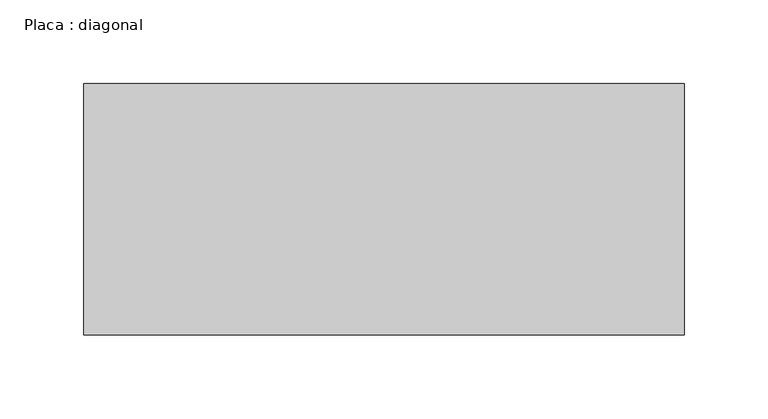
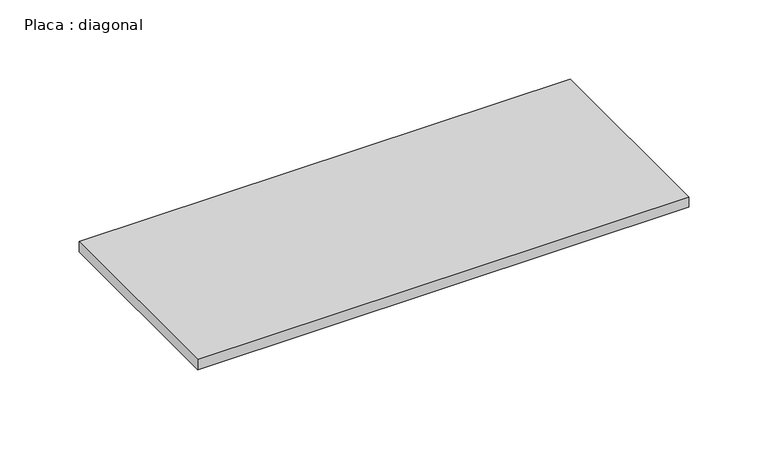
"""IFC4 building model written with IfcOpenShell, lengths in millimetres: beam geometry, Placa : diagonal."""

from ifc_helpers import new_model, si_unit, frame, origin, place, context, project, spatial, polyline, outline, extrude, source, transform, mapped, element, save


def placa_diagonal_6d03bdc5(model_context):
    return source(origin(), model_context, "Body", "SweptSolid", [
        extrude(outline(polyline([(191.209825, 75.0), (191.209825, -75.0), (-166.9394885, -75.0), (-166.9394885, 75.0), (191.209825, 75.0)])), frame((0.0, 0.0, -4.0), z_axis=(0.0, 0.0, 1.0), x_axis=(1.0, 0.0, 0.0)), (0.0, 0.0, 1.0), 8.0),
    ])


if __name__ == "__main__":
    model = new_model("IFC4")
    model_context = context("Model", 3, world=origin())
    ifc_project = project(units=[si_unit("LENGTHUNIT", "METRE", prefix="MILLI")], contexts=[model_context])
    site = spatial("IfcSite", under=ifc_project)
    building = spatial("IfcBuilding", under=site)
    placement = place(None, origin())
    placa_diagonal_shape = placa_diagonal_6d03bdc5(model_context)
    element("IfcBeam", 1, ObjectType="Placa : diagonal", at=placement, inside=building, context=model_context, shape_type="MappedRepresentation", body=[
        mapped(placa_diagonal_shape, transform((0.0, 0.0, 0.0), x_axis=(1.0, 0.0, 0.0), y_axis=(0.0, 1.0, 0.0), z_axis=(0.0, 0.0, 1.0))),
    ])
    save(model, "model.ifc")

# Revit data of these elements
# Type "Placa : diagonal"
#   W = 0
#   Length [instance default] = 1.50 m
#   b = 0.15 m
#   d = 0.008 m
#   A = 0 m²
#   Structural Material [instance default] = Aço, 45-345
# Element 1 (IfcBeam, "Placa : diagonal")
#   Materials on its faces: "Aço, 45-345"
# Materials
#   "Aço, 45-345": class "Metal", colour RGB 247 247 247, transparency 0, Description = "Aço 345 MPa", Cost = 0
